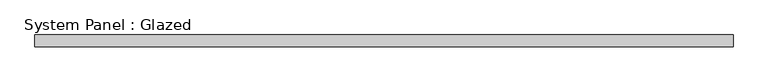
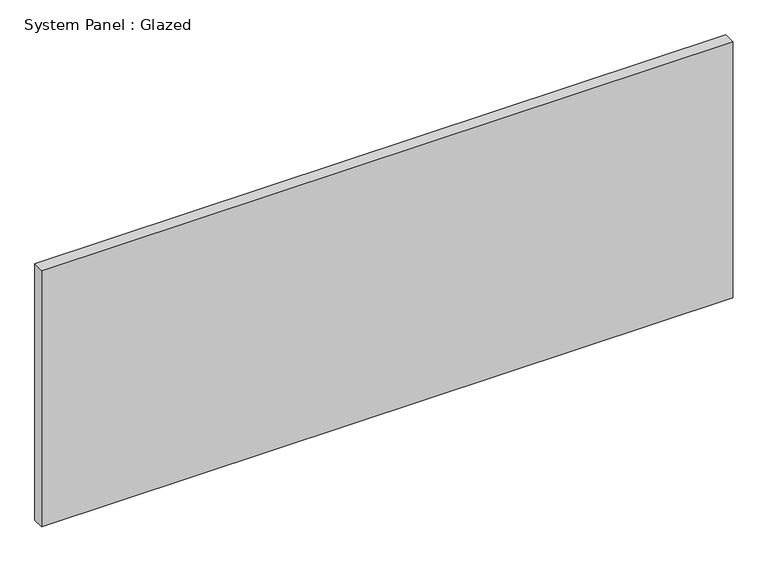
"""IFC4 building model written with IfcOpenShell, lengths in millimetres: plate geometry, System Panel : Glazed."""

from ifc_helpers import new_model, si_unit, origin, origin_with_axes, place, context, project, spatial, polyline, outline, extrude, source, transform, mapped, element, save


def system_panel_glazed_72237fa4(model_context):
    return source(origin(), model_context, "Body", "SweptSolid", [
        extrude(outline(polyline([(762.0, 19.05), (-762.0, 19.05), (-762.0, 44.45), (762.0, 44.45), (762.0, 19.05)])), origin_with_axes(), (0.0, 0.0, 1.0), 596.9),
    ])


if __name__ == "__main__":
    model = new_model("IFC4")
    model_context = context("Model", 3, world=origin())
    ifc_project = project(units=[si_unit("LENGTHUNIT", "METRE", prefix="MILLI")], contexts=[model_context])
    site = spatial("IfcSite", under=ifc_project)
    building = spatial("IfcBuilding", under=site)
    placement = place(None, origin())
    system_panel_glazed_shape = system_panel_glazed_72237fa4(model_context)
    element("IfcPlate", 1, ObjectType="System Panel : Glazed", at=placement, inside=building, context=model_context, shape_type="MappedRepresentation", body=[
        mapped(system_panel_glazed_shape, transform((0.0, 0.0, 0.0), x_axis=(1.0, 0.0, 0.0), y_axis=(0.0, 1.0, 0.0), z_axis=(0.0, 0.0, 1.0))),
    ])
    save(model, "model.ifc")

# Revit data of these elements
# Element 1 (IfcPlate, "System Panel : Glazed")
#   Materials on its faces: "Glass"
# Materials
#   "Glass": class "Glass", colour RGB 0 128 192, transparency 0.75
